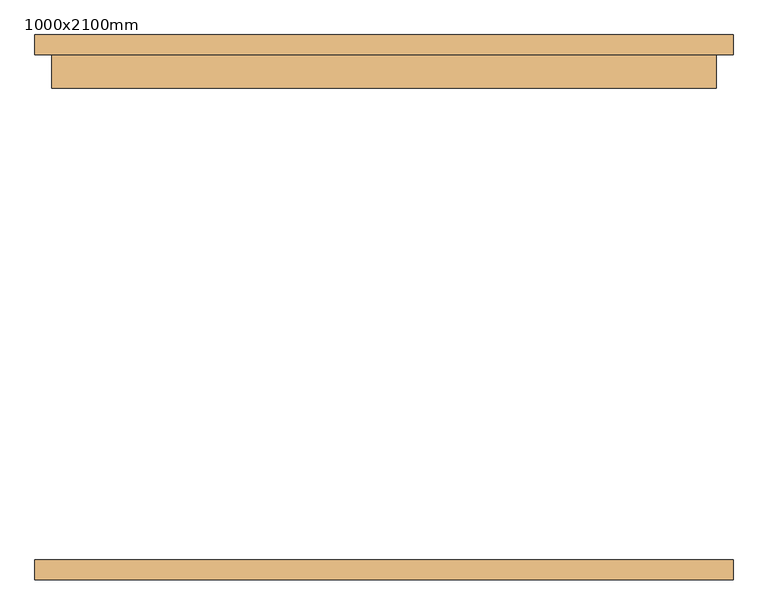
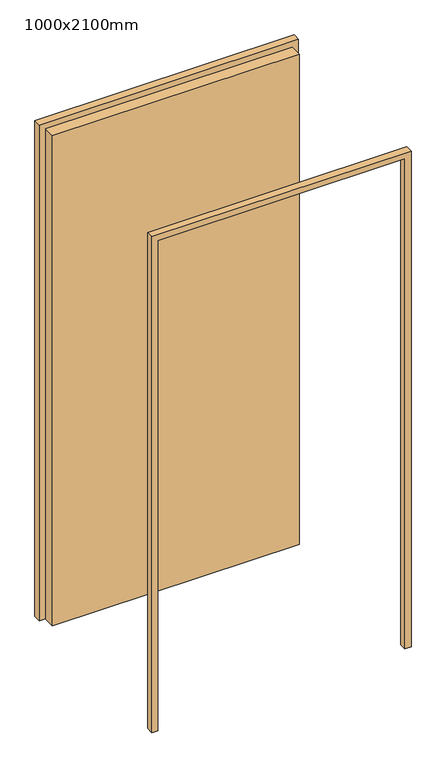
"""IFC4 building model written with IfcOpenShell, lengths in millimetres: door geometry, WWm-SingleSolid-Flush : 1000x2100mm."""

from ifc_helpers import new_model, si_unit, frame, origin, origin_with_axes, place, context, project, spatial, polyline, outline, extrude, source, transform, mapped, element, save


def door_1000x2100mm_209687b1(model_context):
    return source(origin(), model_context, "Body", "SweptSolid", [
        extrude(outline(polyline([(2125.0, -525.0), (0.0, -525.0), (0.0, -500.0), (2100.0, -500.0), (2100.0, 500.0), (0.0, 500.0), (0.0, 525.0), (2125.0, 525.0), (2125.0, -525.0)])), frame((0.0, 380.0, 0.0), z_axis=(0.0, 1.0, 0.0), x_axis=(0.0, 0.0, 1.0)), (0.0, 0.0, 1.0), 30.0),
        extrude(outline(polyline([(2125.0, 525.0), (2125.0, -525.0), (0.0, -525.0), (0.0, -500.0), (2100.0, -500.0), (2100.0, 500.0), (0.0, 500.0), (0.0, 525.0), (2125.0, 525.0)])), frame((0.0, -410.0, 0.0), z_axis=(0.0, 1.0, 0.0), x_axis=(0.0, 0.0, 1.0)), (0.0, 0.0, 1.0), 30.0),
        extrude(outline(polyline([(500.0, 330.0), (-500.0, 330.0), (-500.0, 380.0), (500.0, 380.0), (500.0, 330.0)])), origin_with_axes(), (0.0, 0.0, 1.0), 2100.0),
    ])


if __name__ == "__main__":
    model = new_model("IFC4")
    model_context = context("Model", 3, world=origin())
    ifc_project = project(units=[si_unit("LENGTHUNIT", "METRE", prefix="MILLI")], contexts=[model_context])
    site = spatial("IfcSite", under=ifc_project)
    building = spatial("IfcBuilding", under=site)
    placement = place(None, origin())
    door_1000x2100mm_shape = door_1000x2100mm_209687b1(model_context)
    element("IfcDoor", 1, ObjectType="WWm-SingleSolid-Flush : 1000x2100mm", at=placement, inside=building, context=model_context, shape_type="MappedRepresentation", body=[
        mapped(door_1000x2100mm_shape, transform((0.0, 0.0, 0.0), x_axis=(1.0, 0.0, 0.0), y_axis=(0.0, 1.0, 0.0), z_axis=(0.0, 0.0, 1.0))),
    ])
    save(model, "model.ifc")

# Revit data of these elements
# Type "WWm-SingleSolid-Flush : 1000x2100mm"
#   Type Mark = "EX1-51"
#   Construction Type Id = "MDOOR"
#   Assembly Code = "C1020"
#   Analytic Construction = "Metal"
#   Thickness = 50 mm
#   Thermal Resistance (R) = 0.270117 (m²·K)/W
#   Heat Transfer Coefficient (U) = 3.7021 W/(m²·K)
#   Height = 2100 mm
#   Trim Projection Ext = 30 mm
#   Trim Projection Int = 30 mm
#   Trim Width = 25 mm
#   Width = 1000 mm
#   Not 90 Degree [instance default] = no
#   90 Degree [instance default] = yes
#   Door Material = WW-EC-RGB-White
#   Frame Material = WW-EC-RGB-White
#   Visual Light Transmittance = 0
#   Solar Heat Gain Coefficient = 0
#   Function = (empty or 0)
#   Wall Closure = (empty or 0)
# Element 1 (IfcDoor, "WWm-SingleSolid-Flush : 1000x2100mm")
#   Materials on its faces: "WW-EC-RGB-White"
# Materials
#   "WW-EC-RGB-White": class "Generic", colour RGB 255 255 255, transparency 0, Comments = "If region requests off-white, swith asset color to RGB 231-228-220", Description = "Generic Color", Cost = 0
